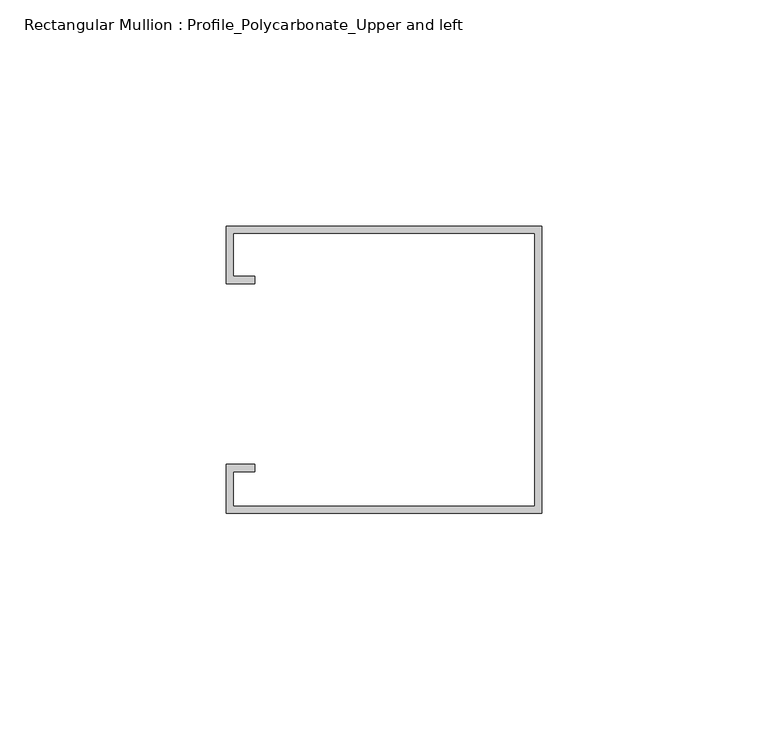
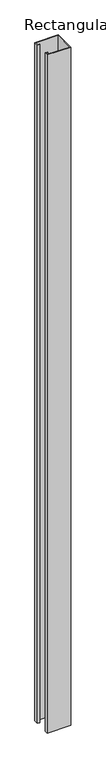
"""IFC4 building model written with IfcOpenShell, lengths in millimetres: member geometry, Rectangular Mullion : Profile_Polycarbonate_Upper and left."""

import ifcopenshell
import ifcopenshell.guid

model = None  # the IFC model being written
_history = None  # IfcOwnerHistory: only IFC2X3 demands one
_inside = {}  # id of a spatial element -> (the spatial element, [elements in it])
_under = {}  # id of a project, library or spatial element -> (it, [spatial elements below it])
_declared = {}  # id of a project -> (the project, [libraries it declares])
_typed = {}  # id of a type object -> (the type object, [elements of that type])
_made_of = {}  # id of a material, layer set ... -> (it, [elements and type objects made of it])


def new_model(schema):
    """Start an empty IFC model of exactly this schema.

    Asked for "IFC4X3", IfcOpenShell would pick the latest addendum, in which some entities
    have other attributes; the version numbers below select the first issue.
    IFC2X3 requires an IfcOwnerHistory on every rooted entity: one is made here for all.
    """
    global model, _history
    if schema == "IFC4X3":
        model = ifcopenshell.file(schema_version=(4, 3, 0, 0))
    else:
        model = ifcopenshell.file(schema=schema)
    _inside.clear()
    _under.clear()
    _declared.clear()
    _typed.clear()
    _made_of.clear()
    _history = None
    if model.schema == "IFC2X3":
        org = make("IfcOrganization", Name="unknown")
        user = make(
            "IfcPersonAndOrganization",
            ThePerson=make("IfcPerson", FamilyName="unknown"),
            TheOrganization=org,
        )
        app = make(
            "IfcApplication",
            ApplicationDeveloper=org,
            Version="unknown",
            ApplicationFullName="unknown",
            ApplicationIdentifier="unknown",
        )
        _history = make(
            "IfcOwnerHistory",
            OwningUser=user,
            OwningApplication=app,
            ChangeAction="ADDED",
            CreationDate=0,
        )
    return model


def make(cls, **values):
    """One entity of the class cls with the attributes given. An attribute that is None is left unset."""
    return model.create_entity(
        cls, **{name: value for name, value in values.items() if value is not None}
    )


def rooted(cls, **values):
    """An entity with a GlobalId (a new one), such as an element, a storey or a relation."""
    return make(cls, GlobalId=ifcopenshell.guid.new(), OwnerHistory=_history, **values)


def si_unit(unit_type, name, prefix=None):
    """IfcSIUnit, for example si_unit("LENGTHUNIT", "METRE", prefix="MILLI")."""
    return make("IfcSIUnit", UnitType=unit_type, Prefix=prefix, Name=name)


def assignment(units):
    """IfcUnitAssignment: the units of a project."""
    return None if units is None else make("IfcUnitAssignment", Units=units)


def point(xyz):
    """IfcCartesianPoint."""
    return None if xyz is None else make("IfcCartesianPoint", Coordinates=xyz)


def direction(xyz):
    """IfcDirection."""
    return None if xyz is None else make("IfcDirection", DirectionRatios=xyz)


def frame(location, z_axis=None, x_axis=None):
    """IfcAxis2Placement3D, a coordinate frame: its origin and axes. An axis left out is left unset."""
    return make(
        "IfcAxis2Placement3D",
        Location=point(location),
        Axis=direction(z_axis),
        RefDirection=direction(x_axis),
    )


def origin():
    """The frame at (0, 0, 0) with its axes left unset."""
    return frame((0.0, 0.0, 0.0))


def place(relative_to, where):
    """IfcLocalPlacement: puts the frame where relative to a parent placement (None: the world)."""
    return make(
        "IfcLocalPlacement", PlacementRelTo=relative_to, RelativePlacement=where
    )


def context(
    kind, dimensions, precision=None, world=None, true_north=None, identifier=None
):
    """IfcGeometricRepresentationContext, for example the 3D "Model" context."""
    return make(
        "IfcGeometricRepresentationContext",
        ContextIdentifier=identifier,
        ContextType=kind,
        CoordinateSpaceDimension=dimensions,
        Precision=precision,
        WorldCoordinateSystem=world,
        TrueNorth=true_north,
    )


def project(units=None, contexts=None):
    """IfcProject with its units and contexts."""
    return rooted(
        "IfcProject",
        Name="project",
        RepresentationContexts=contexts,
        UnitsInContext=assignment(units),
    )


def spatial(cls, under=None, at=None, **own):
    """A site, building, storey or space (cls), placed at a placement, below another one or the project."""
    s = rooted(cls, ObjectPlacement=at, **own)
    if under is not None:
        _under.setdefault(under.id(), (under, []))[1].append(s)
    return s


def polyline(points):
    """IfcPolyline through the points."""
    return make("IfcPolyline", Points=[point(p) for p in points])


def outline(outer, holes=None, kind="AREA"):
    """IfcArbitraryClosedProfileDef: a profile drawn as a closed curve; with holes, ...WithVoids."""
    if holes is None:
        return make("IfcArbitraryClosedProfileDef", ProfileType=kind, OuterCurve=outer)
    return make(
        "IfcArbitraryProfileDefWithVoids",
        ProfileType=kind,
        OuterCurve=outer,
        InnerCurves=holes,
    )


def extrude(swept, where, along, depth):
    """IfcExtrudedAreaSolid: the profile swept, set in the frame where, extruded along a direction by depth."""
    return make(
        "IfcExtrudedAreaSolid",
        SweptArea=swept,
        Position=where,
        ExtrudedDirection=direction(along),
        Depth=depth,
    )


def shape(context_of_items, identifier, shape_type, items):
    """IfcShapeRepresentation: the items that make up one representation, for example the "Body"."""
    return make(
        "IfcShapeRepresentation",
        ContextOfItems=context_of_items,
        RepresentationIdentifier=identifier,
        RepresentationType=shape_type,
        Items=items,
    )


def source(mapping_origin, context_of_items, identifier, shape_type, items):
    """IfcRepresentationMap: a shape defined once, which mapped items show again and again."""
    return make(
        "IfcRepresentationMap",
        MappingOrigin=mapping_origin,
        MappedRepresentation=shape(context_of_items, identifier, shape_type, items),
    )


def transform(
    local_origin,
    x_axis=None,
    y_axis=None,
    z_axis=None,
    scale=None,
    scale2=None,
    scale3=None,
    uniform=True,
):
    """IfcCartesianTransformationOperator3D, or its non-uniform kind. x_axis, y_axis, z_axis: its Axis1, 2, 3."""
    if uniform:
        return make(
            "IfcCartesianTransformationOperator3D",
            Axis1=direction(x_axis),
            Axis2=direction(y_axis),
            LocalOrigin=point(local_origin),
            Scale=scale,
            Axis3=direction(z_axis),
        )
    return make(
        "IfcCartesianTransformationOperator3DnonUniform",
        Axis1=direction(x_axis),
        Axis2=direction(y_axis),
        LocalOrigin=point(local_origin),
        Scale=scale,
        Axis3=direction(z_axis),
        Scale2=scale2,
        Scale3=scale3,
    )


def mapped(mapping_source, mapping_target):
    """IfcMappedItem: shows the shape of a source again, moved by a transform."""
    return make(
        "IfcMappedItem", MappingSource=mapping_source, MappingTarget=mapping_target
    )


def made_of(thing, what):
    """Note that an element or type object is made of a material, layer set ...; save() writes the relation."""
    if what is not None:
        _made_of.setdefault(what.id(), (what, []))[1].append(thing)
    return thing


def element(
    cls,
    number,
    at=None,
    inside=None,
    cuts=None,
    type_object=None,
    material=None,
    context=None,
    identifier="Body",
    shape_type=None,
    held_by="IfcProductDefinitionShape",
    body=None,
    shapes=None,
    **own,
):
    """One element of the class cls, such as IfcWall. Its Tag is "e" and its number.

    at: its placement. inside: the storey or other place that contains it. cuts: it is an
    opening in that element (IfcRelVoidsElement). A single representation is given by context,
    identifier, shape_type and body (its items); several are given by shapes. held_by: the class
    of the entity that holds the representations. save() writes the other relations.
    """
    e = rooted(cls, Tag="e%d" % number, ObjectPlacement=at, **own)
    if body is not None:
        shapes = [shape(context, identifier, shape_type, body)]
    if shapes is not None:
        e.Representation = make(held_by, Representations=shapes)
    if inside is not None:
        _inside.setdefault(inside.id(), (inside, []))[1].append(e)
    if cuts is not None:
        rooted(
            "IfcRelVoidsElement", RelatingBuildingElement=cuts, RelatedOpeningElement=e
        )
    if type_object is not None:
        _typed.setdefault(type_object.id(), (type_object, []))[1].append(e)
    return made_of(e, material)


def aggregate(whole, parts):
    """IfcRelAggregates: a whole, such as a stair, and the parts it consists of."""
    return rooted("IfcRelAggregates", RelatingObject=whole, RelatedObjects=parts)


def save(model, path):
    """Write the relations noted so far, then the file.

    IfcRelAggregates (storeys below a building ...), IfcRelContainedInSpatialStructure (elements
    in a storey), IfcRelDefinesByType, IfcRelAssociatesMaterial and IfcRelDeclares: one each for
    every whole, place, type object, material and project.
    """
    for whole, parts in _under.values():
        aggregate(whole, parts)
    for where, things in _inside.values():
        rooted(
            "IfcRelContainedInSpatialStructure",
            RelatedElements=things,
            RelatingStructure=where,
        )
    for kind, things in _typed.values():
        rooted("IfcRelDefinesByType", RelatedObjects=things, RelatingType=kind)
    for what, things in _made_of.values():
        rooted("IfcRelAssociatesMaterial", RelatedObjects=things, RelatingMaterial=what)
    for by, libraries in _declared.values():
        rooted("IfcRelDeclares", RelatingContext=by, RelatedDefinitions=libraries)
    model.write(path)


def rectangular_mullion_profile_polycarbonate_upper_and_left_535a81d9(model_context):
    return source(origin(), model_context, "Body", "SweptSolid", [
        extrude(outline(polyline([(0.0, 32.7), (0.0, -30.8), (-69.85, -30.8), (-69.85, -20.0), (-63.5, -20.0), (-63.5, -21.5875), (-68.2625, -21.5875), (-68.2625, -29.2125), (-1.5875, -29.2125), (-1.5875, 31.1125), (-68.2625, 31.1125), (-68.2625, 21.5875), (-63.5, 21.5875), (-63.5, 20.0), (-69.85, 20.0), (-69.85, 32.7), (0.0, 32.7)])), frame((0.0, 0.0, -2133.6), z_axis=(0.0, 0.0, 1.0), x_axis=(1.0, 0.0, 0.0)), (0.0, 0.0, 1.0), 2133.6),
    ])


if __name__ == "__main__":
    model = new_model("IFC4")
    model_context = context("Model", 3, world=origin())
    ifc_project = project(units=[si_unit("LENGTHUNIT", "METRE", prefix="MILLI")], contexts=[model_context])
    site = spatial("IfcSite", under=ifc_project)
    building = spatial("IfcBuilding", under=site)
    placement = place(None, origin())
    rectangular_mullion_profile_polycarbonate_upper_and_left_shape = rectangular_mullion_profile_polycarbonate_upper_and_left_535a81d9(model_context)
    element("IfcMember", 1, ObjectType="Rectangular Mullion : Profile_Polycarbonate_Upper and left", at=placement, inside=building, context=model_context, shape_type="MappedRepresentation", body=[
        mapped(rectangular_mullion_profile_polycarbonate_upper_and_left_shape, transform((0.0, 0.0, 0.0), x_axis=(1.0, 0.0, 0.0), y_axis=(0.0, 1.0, 0.0), z_axis=(0.0, 0.0, 1.0))),
    ])
    save(model, "model.ifc")

# Revit data of these elements
# Type "Rectangular Mullion : Profile_Polycarbonate_Upper and left"
#   built-in parameter 1007322 = 0.208333 (stored number, unit not read)
#   built-in parameter 1007321 = 0.00520833 (stored number, unit not read)
#   built-in parameter 1007320 = 0 (stored number, unit not read)
# Element 1 (IfcMember, "Rectangular Mullion : Profile_Polycarbonate_Upper and left")
#   Materials on its faces: "ALUMINUM PROFILE AT POLYCARBONATE PANEL"
# Materials
#   "ALUMINUM PROFILE AT POLYCARBONATE PANEL": class "Metal", colour RGB 244 244 244, transparency 0, Description = "Aluminum 6061", Cost = 0
